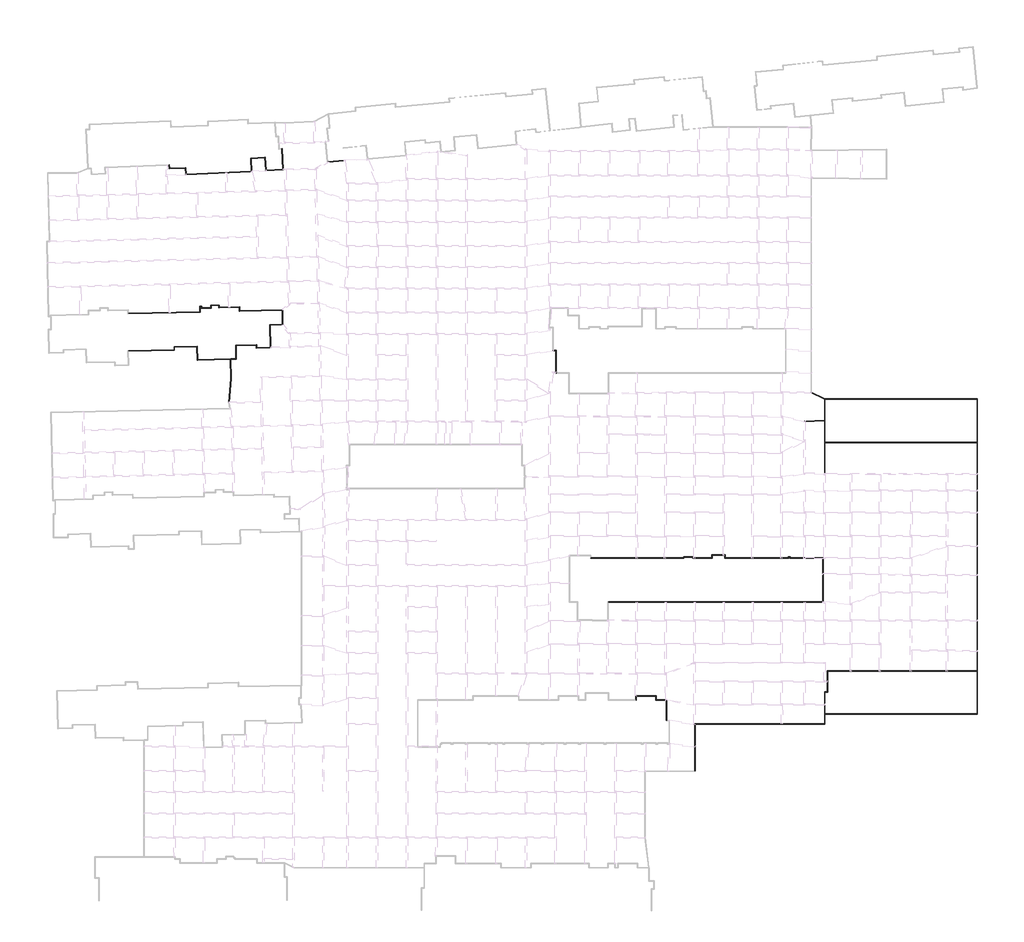
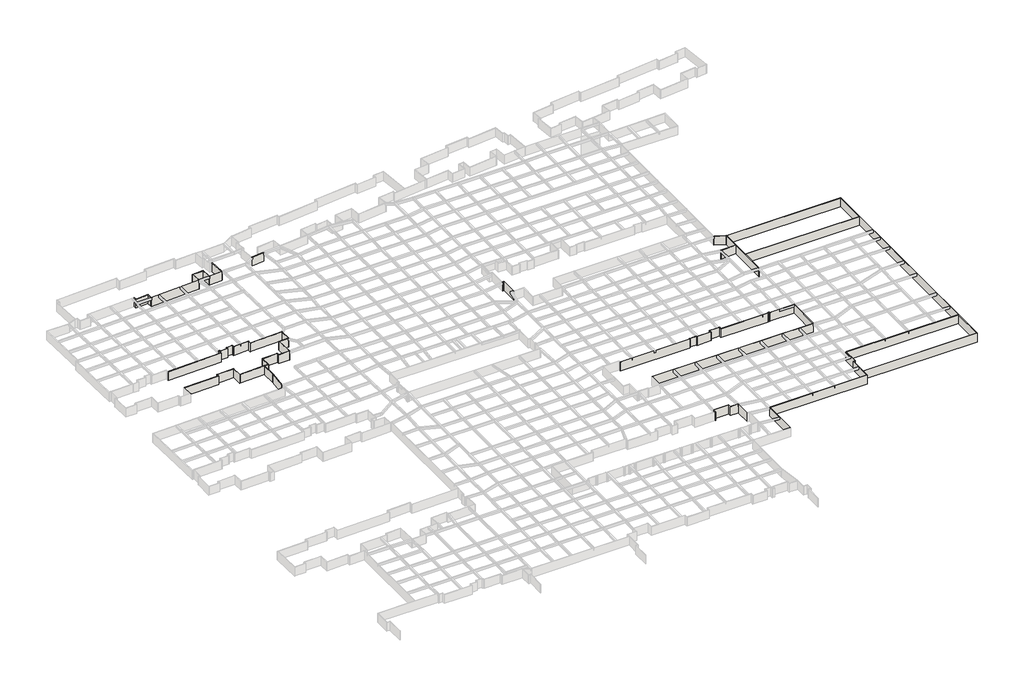
# One storey, part 5 of 20: 71 walls.
"""IFC4 building model written with IfcOpenShell, lengths in millimetres."""

from ifc_helpers import new_model, si_unit, origin, origin_with_axes, place, context, project, spatial, polyline, outline, extrude, faceted_brep, element, save

model = new_model("IFC4")

# Units and contexts
model_context = context("Model", 3, world=origin())
ifc_project = project(units=[si_unit("LENGTHUNIT", "METRE", prefix="MILLI")], contexts=[model_context])

# Site, building, storey
site = spatial("IfcSite", under=ifc_project)
building = spatial("IfcBuilding", under=site)
storey = spatial("IfcBuildingStorey", under=building, Name="户型图", Elevation=0.0)

# Walls
placement = place(None, origin())
element("IfcWall", 1, ObjectType="所有墙体", at=placement, inside=storey, context=model_context, shape_type="Brep", body=[
    faceted_brep([(-4228.4021072, 138757.8636225, 0.0), (8173.0072094, 139059.136348, 0.0), (8173.0072094, 139059.136348, 3300.0), (-4228.4021072, 138757.8636225, 3300.0), (-4231.3164585, 138877.8282279, 0.0), (-4231.3164585, 138877.8282279, 3300.0), (8053.0072094, 139176.2565418, 3300.0), (8173.0072094, 139179.171753, 3300.0), (8173.0072094, 139179.171753, 0.0), (8053.0072094, 139176.2565418, 0.0)], [[[0, 1, 2, 3]], [[4, 5, 6, 7, 8, 9]], [[1, 0, 4, 9, 8]], [[3, 2, 7, 6, 5]], [[0, 3, 5, 4]], [[2, 1, 8, 7]]]),
])
element("IfcWall", 2, ObjectType="所有墙体", at=placement, inside=storey, context=model_context, shape_type="Brep", body=[
    faceted_brep([(8173.0072094, 139179.171753, 0.0), (8173.0072094, 139859.136348, 0.0), (8173.0072094, 139979.171753, 0.0), (8173.0072094, 139979.171753, 3300.0), (8173.0072094, 139859.136348, 3300.0), (8173.0072094, 139179.171753, 3300.0), (8053.0072094, 139176.2565418, 0.0), (8053.0072094, 139176.2565418, 3300.0), (8053.0072094, 139976.2565418, 3300.0), (8053.0072094, 139976.2565418, 0.0)], [[[0, 1, 2, 3, 4, 5]], [[6, 7, 8, 9]], [[2, 1, 0, 6, 9]], [[5, 4, 3, 8, 7]], [[0, 5, 7, 6]], [[3, 2, 9, 8]]]),
])
element("IfcWall", 3, ObjectType="所有墙体", at=placement, inside=storey, context=model_context, shape_type="Brep", body=[
    faceted_brep([(8173.0072094, 139859.136348, 0.0), (14152.6828585, 140004.4031588, 0.0), (14272.6474639, 140007.3175101, 0.0), (14272.6474639, 140007.3175101, 3300.0), (14152.6828585, 140004.4031588, 3300.0), (8173.0072094, 139859.136348, 3300.0), (8173.0072094, 139979.171753, 0.0), (8173.0072094, 139979.171753, 3300.0), (14269.7331126, 140127.2821155, 3300.0), (14269.7331126, 140127.2821155, 0.0)], [[[0, 1, 2, 3, 4, 5]], [[6, 7, 8, 9]], [[2, 1, 0, 6, 9]], [[5, 4, 3, 8, 7]], [[0, 5, 7, 6]], [[3, 2, 9, 8]]]),
])
element("IfcWall", 4, ObjectType="所有墙体", at=placement, inside=storey, context=model_context, shape_type="Brep", body=[
    faceted_brep([(14152.6828585, 140004.4031588, 0.0), (14240.0810776, 136406.7954185, 0.0), (14240.0810776, 136406.7954185, 3300.0), (14152.6828585, 140004.4031588, 3300.0), (14272.6474639, 140007.3175101, 0.0), (14272.6474639, 140007.3175101, 3300.0), (14357.1313318, 136529.6743753, 3300.0), (14360.0456831, 136409.7097698, 3300.0), (14360.0456831, 136409.7097698, 0.0), (14357.1313318, 136529.6743753, 0.0)], [[[0, 1, 2, 3]], [[4, 5, 6, 7, 8, 9]], [[1, 0, 4, 9, 8]], [[3, 2, 7, 6, 5]], [[0, 3, 5, 4]], [[2, 1, 8, 7]]]),
])
element("IfcWall", 5, ObjectType="所有墙体", at=placement, inside=storey, context=model_context, shape_type="Brep", body=[
    faceted_brep([(14360.0456831, 136409.7097698, 0.0), (23216.491821, 136624.863193, 0.0), (23336.4564264, 136627.7775443, 0.0), (23336.4564264, 136627.7775443, 3300.0), (23216.491821, 136624.863193, 3300.0), (14360.0456831, 136409.7097698, 3300.0), (14357.1313318, 136529.6743753, 0.0), (14357.1313318, 136529.6743753, 3300.0), (23246.0635256, 136745.616996, 3300.0), (23333.5420751, 136747.7421497, 3300.0), (23333.5420751, 136747.7421497, 0.0), (23246.0635256, 136745.616996, 0.0), (23335.6240877, 136662.0394333, 0.0), (23335.6240877, 136662.0394333, 3300.0)], [[[0, 1, 2, 3, 4, 5]], [[6, 7, 8, 9, 10, 11]], [[2, 1, 0, 6, 11, 10, 12]], [[5, 4, 3, 13, 9, 8, 7]], [[0, 5, 7, 6]], [[3, 2, 12, 10, 9, 13]]]),
])
element("IfcWall", 6, ObjectType="所有墙体", at=placement, inside=storey, context=model_context, shape_type="SweptSolid", body=[
    extrude(outline(polyline([(23339.7846649, 131549.7107032), (23216.491821, 136624.863193), (23336.4564264, 136627.7775443), (23459.9119945, 131545.9267742), (23339.7846649, 131549.7107032)])), origin_with_axes(), (0.0, 0.0, 1.0), 3300.0),
])
element("IfcWall", 7, ObjectType="所有墙体", at=placement, inside=storey, context=model_context, shape_type="SweptSolid", body=[
    extrude(outline(polyline([(22764.2529371, 124971.3529529), (23339.7846649, 131549.7107032), (23459.9119945, 131545.9267742), (22884.987918, 124974.5145097), (22764.2529371, 124971.3529529)])), origin_with_axes(), (0.0, 0.0, 1.0), 3300.0),
])
element("IfcWall", 8, ObjectType="所有墙体", at=placement, inside=storey, context=model_context, shape_type="Brep", body=[
    faceted_brep([(148100.0, 25994.6126828, 0.0), (148100.0, 38580.0, 0.0), (148100.0, 38700.0, 0.0), (148100.0, 38700.0, 3300.0), (148100.0, 38580.0, 3300.0), (148100.0, 25994.6126828, 3300.0), (147980.0, 25994.6126828, 0.0), (147980.0, 25994.6126828, 3300.0), (147980.0, 38700.0, 3300.0), (147980.0, 38700.0, 0.0)], [[[0, 1, 2, 3, 4, 5]], [[6, 7, 8, 9]], [[2, 1, 0, 6, 9]], [[5, 4, 3, 8, 7]], [[0, 5, 7, 6]], [[3, 2, 9, 8]]]),
])
element("IfcWall", 9, ObjectType="所有墙体", at=placement, inside=storey, context=model_context, shape_type="Brep", body=[
    faceted_brep([(148100.0, 38580.0, 0.0), (182984.9999996, 38580.0, 0.0), (182984.9999996, 38580.0, 3300.0), (148100.0, 38580.0, 3300.0), (148100.0, 38700.0, 0.0), (148100.0, 38700.0, 3300.0), (182864.9999996, 38700.0, 3300.0), (182984.9999996, 38700.0, 3300.0), (182984.9999996, 38700.0, 0.0), (182864.9999996, 38700.0, 0.0)], [[[0, 1, 2, 3]], [[4, 5, 6, 7, 8, 9]], [[1, 0, 4, 9, 8]], [[3, 2, 7, 6, 5]], [[0, 3, 5, 4]], [[2, 1, 8, 7]]]),
])
element("IfcWall", 10, ObjectType="所有墙体", at=placement, inside=storey, context=model_context, shape_type="Brep", body=[
    faceted_brep([(182984.9999996, 38700.0, 0.0), (182984.9999996, 41206.0, 0.0), (182984.9999996, 41326.0, 0.0), (182984.9999996, 47205.0, 0.0), (182984.9999996, 47325.0, 0.0), (182984.9999996, 47325.0, 3300.0), (182984.9999996, 47205.0, 3300.0), (182984.9999996, 41326.0, 3300.0), (182984.9999996, 41206.0, 3300.0), (182984.9999996, 38700.0, 3300.0), (182864.9999996, 38700.0, 0.0), (182864.9999996, 38700.0, 3300.0), (182864.9999996, 47325.0, 3300.0), (182864.9999996, 47325.0, 0.0)], [[[0, 1, 2, 3, 4, 5, 6, 7, 8, 9]], [[10, 11, 12, 13]], [[4, 3, 2, 1, 0, 10, 13]], [[9, 8, 7, 6, 5, 12, 11]], [[0, 9, 11, 10]], [[5, 4, 13, 12]]]),
])
element("IfcWall", 11, ObjectType="所有墙体", at=placement, inside=storey, context=model_context, shape_type="Brep", body=[
    faceted_brep([(182984.9999996, 41206.0, 0.0), (223958.0, 41206.0, 0.0), (223958.0, 41206.0, 3300.0), (182984.9999996, 41206.0, 3300.0), (182984.9999996, 41326.0, 0.0), (182984.9999996, 41326.0, 3300.0), (223838.0, 41326.0, 3300.0), (223958.0, 41326.0, 3300.0), (223958.0, 41326.0, 0.0), (223838.0, 41326.0, 0.0)], [[[0, 1, 2, 3]], [[4, 5, 6, 7, 8, 9]], [[1, 0, 4, 9, 8]], [[3, 2, 7, 6, 5]], [[0, 3, 5, 4]], [[2, 1, 8, 7]]]),
])
element("IfcWall", 12, ObjectType="所有墙体", at=placement, inside=storey, context=model_context, shape_type="Brep", body=[
    faceted_brep([(223958.0, 41326.0, 0.0), (223958.0, 126084.0, 0.0), (223958.0, 126084.0, 3300.0), (223958.0, 41326.0, 3300.0), (223838.0, 41326.0, 0.0), (223838.0, 41326.0, 3300.0), (223838.0, 52805.0, 3300.0), (223838.0, 52925.0, 3300.0), (223838.0, 114264.0, 3300.0), (223838.0, 114384.0, 3300.0), (223838.0, 125964.0, 3300.0), (223838.0, 126084.0, 3300.0), (223838.0, 126084.0, 0.0), (223838.0, 125964.0, 0.0), (223838.0, 114384.0, 0.0), (223838.0, 114264.0, 0.0), (223838.0, 52925.0, 0.0), (223838.0, 52805.0, 0.0)], [[[0, 1, 2, 3]], [[4, 5, 6, 7, 8, 9, 10, 11, 12, 13, 14, 15, 16, 17]], [[1, 0, 4, 17, 16, 15, 14, 13, 12]], [[3, 2, 11, 10, 9, 8, 7, 6, 5]], [[0, 3, 5, 4]], [[2, 1, 12, 11]]]),
])
element("IfcWall", 13, ObjectType="所有墙体", at=placement, inside=storey, context=model_context, shape_type="Brep", body=[
    faceted_brep([(223838.0, 126084.0, 0.0), (182938.3016794, 126084.0, 0.0), (182654.3574894, 126084.0, 0.0), (182654.3574894, 126084.0, 3300.0), (182938.3016794, 126084.0, 3300.0), (223838.0, 126084.0, 3300.0), (223838.0, 125964.0, 0.0), (223838.0, 125964.0, 3300.0), (182984.9999996, 125964.0, 3300.0), (182911.6983199, 125964.0, 3300.0), (182911.6983199, 125964.0, 0.0), (182984.9999996, 125964.0, 0.0), (182864.9999996, 125985.7757844, 0.0), (182864.9999996, 125985.7757844, 3300.0)], [[[0, 1, 2, 3, 4, 5]], [[6, 7, 8, 9, 10, 11]], [[2, 1, 0, 6, 11, 10, 12]], [[5, 4, 3, 13, 9, 8, 7]], [[0, 5, 7, 6]], [[3, 2, 12, 10, 9, 13]]]),
])
element("IfcWall", 14, ObjectType="所有墙体", at=placement, inside=storey, context=model_context, shape_type="Brep", body=[
    faceted_brep([(182938.3016794, 126084.0, 0.0), (179359.7688515, 127752.6972626, 0.0), (179239.7688515, 127808.6541816, 0.0), (179239.7688515, 127808.6541816, 3300.0), (179359.7688515, 127752.6972626, 3300.0), (182938.3016794, 126084.0, 3300.0), (182654.3574894, 126084.0, 0.0), (182654.3574894, 126084.0, 3300.0), (179239.7688515, 127676.2488313, 3300.0), (179239.7688515, 127676.2488313, 0.0)], [[[0, 1, 2, 3, 4, 5]], [[6, 7, 8, 9]], [[2, 1, 0, 6, 9]], [[5, 4, 3, 8, 7]], [[0, 5, 7, 6]], [[3, 2, 9, 8]]]),
])
element("IfcWall", 15, ObjectType="所有墙体", at=placement, inside=storey, context=model_context, shape_type="SweptSolid", body=[
    extrude(outline(polyline([(53846.8616542, 190018.1389708), (49331.2355692, 189543.5275444), (49319.6896824, 189662.9750163), (53834.3182386, 190137.4815982), (53846.8616542, 190018.1389708)])), origin_with_axes(), (0.0, 0.0, 1.0), 3300.0),
])
element("IfcWall", 16, ObjectType="所有墙体", at=placement, inside=storey, context=model_context, shape_type="Brep", body=[
    faceted_brep([(37019.504808, 193167.4722862, 0.0), (37309.4460056, 187635.0646637, 0.0), (37315.7263203, 187515.2291195, 0.0), (37315.7263203, 187515.2291195, 3300.0), (37309.4460056, 187635.0646637, 3300.0), (37019.504808, 193167.4722862, 3300.0), (37139.3403522, 193173.752601, 0.0), (37139.3403522, 193173.752601, 3300.0), (37435.5618645, 187521.5094342, 3300.0), (37435.5618645, 187521.5094342, 0.0)], [[[0, 1, 2, 3, 4, 5]], [[6, 7, 8, 9]], [[2, 1, 0, 6, 9]], [[5, 4, 3, 8, 7]], [[0, 5, 7, 6]], [[3, 2, 9, 8]]]),
])
element("IfcWall", 17, ObjectType="所有墙体", at=placement, inside=storey, context=model_context, shape_type="Brep", body=[
    faceted_brep([(37309.4460056, 187635.0646637, 0.0), (32786.9007673, 187398.048111, 0.0), (32667.0652231, 187391.7677963, 0.0), (32667.0652231, 187391.7677963, 3300.0), (32786.9007673, 187398.048111, 3300.0), (37309.4460056, 187635.0646637, 3300.0), (37315.7263203, 187515.2291195, 0.0), (37315.7263203, 187515.2291195, 3300.0), (32793.1810821, 187278.2125669, 3300.0), (32673.3455379, 187271.9322521, 3300.0), (32673.3455379, 187271.9322521, 2500.0), (32673.3455379, 187271.9322521, 0.0)], [[[0, 1, 2, 3, 4, 5]], [[6, 7, 8, 9, 10, 11]], [[2, 1, 0, 6, 11]], [[5, 4, 3, 9, 8, 7]], [[0, 5, 7, 6]], [[3, 2, 11, 10, 9]]]),
])
element("IfcWall", 18, ObjectType="所有墙体", at=placement, inside=storey, context=model_context, shape_type="Brep", body=[
    faceted_brep([(32786.9007673, 187398.048111, 0.0), (32602.4342162, 190917.8795872, 0.0), (32602.4342162, 190917.8795872, 3300.0), (32786.9007673, 187398.048111, 3300.0), (32667.0652231, 187391.7677963, 0.0), (32667.0652231, 187391.7677963, 3300.0), (32488.8789868, 190791.7637283, 3300.0), (32482.598672, 190911.5992725, 3300.0), (32482.598672, 190911.5992725, 0.0), (32488.8789868, 190791.7637283, 0.0)], [[[0, 1, 2, 3]], [[4, 5, 6, 7, 8, 9]], [[1, 0, 4, 9, 8]], [[3, 2, 7, 6, 5]], [[0, 3, 5, 4]], [[2, 1, 8, 7]]]),
])
element("IfcWall", 19, ObjectType="所有墙体", at=placement, inside=storey, context=model_context, shape_type="Brep", body=[
    faceted_brep([(32482.598672, 190911.5992725, 0.0), (28607.9160772, 190708.5357622, 0.0), (28607.9160772, 190708.5357622, 3300.0), (32482.598672, 190911.5992725, 3300.0), (32488.8789868, 190791.7637283, 0.0), (32488.8789868, 190791.7637283, 3300.0), (28734.0319361, 190594.9805328, 3300.0), (28614.1963919, 190588.7002181, 3300.0), (28614.1963919, 190588.7002181, 0.0), (28734.0319361, 190594.9805328, 0.0)], [[[0, 1, 2, 3]], [[4, 5, 6, 7, 8, 9]], [[1, 0, 4, 9, 8]], [[3, 2, 7, 6, 5]], [[0, 3, 5, 4]], [[2, 1, 8, 7]]]),
])
element("IfcWall", 20, ObjectType="所有墙体", at=placement, inside=storey, context=model_context, shape_type="Brep", body=[
    faceted_brep([(28614.1963919, 190588.7002181, 0.0), (28794.7279523, 187143.9528373, 0.0), (28801.0084588, 187024.1136344, 0.0), (28801.0084588, 187024.1136344, 3300.0), (28794.7279523, 187143.9528373, 3300.0), (28614.1963919, 190588.7002181, 3300.0), (28734.0319361, 190594.9805328, 0.0), (28734.0319361, 190594.9805328, 3300.0), (28920.893079, 187029.4575233, 3300.0), (28920.893079, 187029.4575233, 0.0)], [[[0, 1, 2, 3, 4, 5]], [[6, 7, 8, 9]], [[2, 1, 0, 6, 9]], [[5, 4, 3, 8, 7]], [[0, 5, 7, 6]], [[3, 2, 9, 8]]]),
])
element("IfcWall", 21, ObjectType="所有墙体", at=placement, inside=storey, context=model_context, shape_type="Brep", body=[
    faceted_brep([(28794.7279523, 187143.9528373, 0.0), (11317.4343518, 186364.8978146, 0.0), (11197.5533917, 186359.5540888, 0.0), (11197.5533917, 186359.5540888, 3300.0), (11317.4343518, 186364.8978146, 3300.0), (28794.7279523, 187143.9528373, 3300.0), (28801.0084588, 187024.1136344, 0.0), (28801.0084588, 187024.1136344, 3300.0), (11322.7780776, 186245.0168545, 3300.0), (11202.8971175, 186239.6731287, 3300.0), (11202.8971175, 186239.6731287, 2500.0), (11202.8971175, 186239.6731287, 0.0)], [[[0, 1, 2, 3, 4, 5]], [[6, 7, 8, 9, 10, 11]], [[2, 1, 0, 6, 11]], [[5, 4, 3, 9, 8, 7]], [[0, 5, 7, 6]], [[3, 2, 11, 10, 9]]]),
])
element("IfcWall", 22, ObjectType="所有墙体", at=placement, inside=storey, context=model_context, shape_type="Brep", body=[
    faceted_brep([(11317.4343518, 186364.8978146, 0.0), (11237.3451707, 188161.6157523, 0.0), (11237.3451707, 188161.6157523, 3300.0), (11317.4343518, 186364.8978146, 3300.0), (11197.5533917, 186359.5540888, 0.0), (11197.5533917, 186359.5540888, 3300.0), (11122.8079363, 188036.3910664, 3300.0), (11117.4642106, 188156.2720265, 3300.0), (11117.4642106, 188156.2720265, 0.0), (11122.8079363, 188036.3910664, 0.0)], [[[0, 1, 2, 3]], [[4, 5, 6, 7, 8, 9]], [[1, 0, 4, 9, 8]], [[3, 2, 7, 6, 5]], [[0, 3, 5, 4]], [[2, 1, 8, 7]]]),
])
element("IfcWall", 23, ObjectType="所有墙体", at=placement, inside=storey, context=model_context, shape_type="Brep", body=[
    faceted_brep([(11117.4642106, 188156.2720265, 0.0), (6836.276518, 187965.4369435, 0.0), (6716.3955579, 187960.0932177, 0.0), (6716.3955579, 187960.0932177, 3300.0), (6836.276518, 187965.4369435, 3300.0), (11117.4642106, 188156.2720265, 3300.0), (11122.8079363, 188036.3910664, 0.0), (11122.8079363, 188036.3910664, 3300.0), (6721.7392837, 187840.2122576, 3300.0), (6721.7392837, 187840.2122576, 0.0)], [[[0, 1, 2, 3, 4, 5]], [[6, 7, 8, 9]], [[2, 1, 0, 6, 9]], [[5, 4, 3, 8, 7]], [[0, 5, 7, 6]], [[3, 2, 9, 8]]]),
])
element("IfcWall", 24, ObjectType="所有墙体", at=placement, inside=storey, context=model_context, shape_type="Brep", body=[
    faceted_brep([(6836.276518, 187965.4369435, 0.0), (6791.7370894, 188964.6329557, 0.0), (6791.7370894, 188964.6329557, 3300.0), (6836.276518, 187965.4369435, 3300.0), (6716.3955579, 187960.0932177, 0.0), (6716.3955579, 187960.0932177, 3300.0), (6677.199855, 188839.4082698, 3300.0), (6671.8561293, 188959.2892299, 3300.0), (6671.8561293, 188959.2892299, 0.0), (6677.199855, 188839.4082698, 0.0)], [[[0, 1, 2, 3]], [[4, 5, 6, 7, 8, 9]], [[1, 0, 4, 9, 8]], [[3, 2, 7, 6, 5]], [[0, 3, 5, 4]], [[2, 1, 8, 7]]]),
])
element("IfcWall", 25, ObjectType="所有墙体", at=placement, inside=storey, context=model_context, shape_type="Brep", body=[
    faceted_brep([(109995.8712071, 138929.7156576, 0.0), (110579.0, 138929.7156576, 0.0), (110699.0, 138929.7156576, 0.0), (110699.0, 138929.7156576, 3300.0), (110579.0, 138929.7156576, 3300.0), (109995.8712071, 138929.7156576, 3300.0), (109995.8712071, 139049.7156576, 0.0), (109995.8712071, 139049.7156576, 3300.0), (110699.0, 139049.7156576, 3300.0), (110699.0, 139049.7156576, 0.0)], [[[0, 1, 2, 3, 4, 5]], [[6, 7, 8, 9]], [[2, 1, 0, 6, 9]], [[5, 4, 3, 8, 7]], [[0, 5, 7, 6]], [[3, 2, 9, 8]]]),
])
element("IfcWall", 26, ObjectType="所有墙体", at=placement, inside=storey, context=model_context, shape_type="Brep", body=[
    faceted_brep([(110579.0, 138929.7156576, 0.0), (110579.0, 132933.0, 0.0), (110579.0, 132933.0, 3300.0), (110579.0, 138929.7156576, 3300.0), (110699.0, 138929.7156576, 0.0), (110699.0, 138929.7156576, 3300.0), (110699.0, 133053.0, 3300.0), (110699.0, 132933.0, 3300.0), (110699.0, 132933.0, 0.0), (110699.0, 133053.0, 0.0)], [[[0, 1, 2, 3]], [[4, 5, 6, 7, 8, 9]], [[1, 0, 4, 9, 8]], [[3, 2, 7, 6, 5]], [[0, 3, 5, 4]], [[2, 1, 8, 7]]]),
])
element("IfcWall", 27, ObjectType="所有墙体", at=placement, inside=storey, context=model_context, shape_type="Brep", body=[
    faceted_brep([(182864.9999996, 125985.7757844, 0.0), (182864.9999996, 120234.5396241, 0.0), (182864.9999996, 120114.471487, 0.0), (182864.9999996, 105802.5076858, 0.0), (182864.9999996, 105802.5076858, 3300.0), (182864.9999996, 120114.471487, 3300.0), (182864.9999996, 120234.5396241, 3300.0), (182864.9999996, 125985.7757844, 3300.0), (182984.9999996, 125964.0, 0.0), (182984.9999996, 125964.0, 3300.0), (182984.9999996, 114384.0, 3300.0), (182984.9999996, 114264.0, 3300.0), (182984.9999996, 105802.5076858, 3300.0), (182984.9999996, 105802.5076858, 0.0), (182984.9999996, 114264.0, 0.0), (182984.9999996, 114384.0, 0.0), (182911.6983199, 125964.0, 0.0), (182911.6983199, 125964.0, 3300.0)], [[[0, 1, 2, 3, 4, 5, 6, 7]], [[8, 9, 10, 11, 12, 13, 14, 15]], [[3, 2, 1, 0, 16, 8, 15, 14, 13]], [[4, 3, 13, 12]], [[7, 6, 5, 4, 12, 11, 10, 9, 17]], [[0, 7, 17, 16]], [[17, 9, 8, 16]]]),
])
element("IfcWall", 28, ObjectType="所有墙体", at=placement, inside=storey, context=model_context, shape_type="SweptSolid", body=[
    extrude(outline(polyline([(223838.0, 114264.0), (182984.9999996, 114264.0), (182984.9999996, 114384.0), (223838.0, 114384.0), (223838.0, 114264.0)])), origin_with_axes(), (0.0, 0.0, 1.0), 3300.0),
])
element("IfcWall", 29, ObjectType="所有墙体", at=placement, inside=storey, context=model_context, shape_type="SweptSolid", body=[
    extrude(outline(polyline([(182864.9999996, 120114.471487), (177452.0210746, 119932.0340492), (177447.9789254, 120051.9659508), (182864.9999996, 120234.5396241), (182864.9999996, 120114.471487)])), origin_with_axes(), (0.0, 0.0, 1.0), 3300.0),
])
element("IfcWall", 30, ObjectType="所有墙体", at=placement, inside=storey, context=model_context, shape_type="Brep", body=[
    faceted_brep([(124710.0, 71310.0, 0.0), (182496.0, 71310.0, 0.0), (182496.0, 71310.0, 3300.0), (124710.0, 71310.0, 3300.0), (124710.0, 71430.0, 0.0), (124710.0, 71430.0, 3300.0), (182376.0, 71430.0, 3300.0), (182496.0, 71430.0, 3300.0), (182496.0, 71430.0, 0.0), (182376.0, 71430.0, 0.0)], [[[0, 1, 2, 3]], [[4, 5, 6, 7, 8, 9]], [[1, 0, 4, 9, 8]], [[3, 2, 7, 6, 5]], [[0, 3, 5, 4]], [[2, 1, 8, 7]]]),
])
element("IfcWall", 31, ObjectType="所有墙体", at=placement, inside=storey, context=model_context, shape_type="Brep", body=[
    faceted_brep([(182496.0, 71430.0, 0.0), (182496.0, 83280.0, 0.0), (182496.0, 83280.0, 3300.0), (182496.0, 71430.0, 3300.0), (182376.0, 71430.0, 0.0), (182376.0, 71430.0, 3300.0), (182376.0, 83160.0, 3300.0), (182376.0, 83280.0, 3300.0), (182376.0, 83280.0, 0.0), (182376.0, 83160.0, 0.0)], [[[0, 1, 2, 3]], [[4, 5, 6, 7, 8, 9]], [[1, 0, 4, 9, 8]], [[3, 2, 7, 6, 5]], [[0, 3, 5, 4]], [[2, 1, 8, 7]]]),
])
element("IfcWall", 32, ObjectType="所有墙体", at=placement, inside=storey, context=model_context, shape_type="SweptSolid", body=[
    extrude(outline(polyline([(173697.0, 83280.0), (182376.0, 83280.0), (182376.0, 83160.0), (173697.0, 83160.0), (173697.0, 83280.0)])), origin_with_axes(), (0.0, 0.0, 1.0), 3300.0),
])
element("IfcWall", 33, ObjectType="所有墙体", at=placement, inside=storey, context=model_context, shape_type="Brep", body=[
    faceted_brep([(173697.0, 83160.0, 0.0), (173697.0, 83280.0, 0.0), (173697.0, 83530.0, 0.0), (173697.0, 83530.0, 3300.0), (173697.0, 83280.0, 3300.0), (173697.0, 83160.0, 3300.0), (173577.0, 83160.0, 0.0), (173577.0, 83160.0, 3300.0), (173577.0, 83410.0, 3300.0), (173577.0, 83530.0, 3300.0), (173577.0, 83530.0, 0.0), (173577.0, 83410.0, 0.0)], [[[0, 1, 2, 3, 4, 5]], [[6, 7, 8, 9, 10, 11]], [[2, 1, 0, 6, 11, 10]], [[5, 4, 3, 9, 8, 7]], [[0, 5, 7, 6]], [[3, 2, 10, 9]]]),
])
element("IfcWall", 34, ObjectType="所有墙体", at=placement, inside=storey, context=model_context, shape_type="SweptSolid", body=[
    extrude(outline(polyline([(173197.0, 83530.0), (173577.0, 83530.0), (173577.0, 83410.0), (173197.0, 83410.0), (173197.0, 83530.0)])), origin_with_axes(), (0.0, 0.0, 1.0), 3300.0),
])
element("IfcWall", 35, ObjectType="所有墙体", at=placement, inside=storey, context=model_context, shape_type="Brep", body=[
    faceted_brep([(173077.0, 83530.0, 0.0), (173077.0, 83280.0, 0.0), (173077.0, 83160.0, 0.0), (173077.0, 83160.0, 3300.0), (173077.0, 83280.0, 3300.0), (173077.0, 83530.0, 3300.0), (173197.0, 83530.0, 0.0), (173197.0, 83530.0, 3300.0), (173197.0, 83410.0, 3300.0), (173197.0, 83160.0, 3300.0), (173197.0, 83160.0, 0.0), (173197.0, 83410.0, 0.0)], [[[0, 1, 2, 3, 4, 5]], [[6, 7, 8, 9, 10, 11]], [[2, 1, 0, 6, 11, 10]], [[5, 4, 3, 9, 8, 7]], [[0, 5, 7, 6]], [[3, 2, 10, 9]]]),
])
element("IfcWall", 36, ObjectType="所有墙体", at=placement, inside=storey, context=model_context, shape_type="Brep", body=[
    faceted_brep([(173077.0, 83280.0, 0.0), (156196.0, 83280.0, 0.0), (156076.0, 83280.0, 0.0), (156076.0, 83280.0, 3300.0), (156196.0, 83280.0, 3300.0), (173077.0, 83280.0, 3300.0), (173077.0, 83160.0, 0.0), (173077.0, 83160.0, 3300.0), (156076.0, 83160.0, 3300.0), (156076.0, 83160.0, 0.0)], [[[0, 1, 2, 3, 4, 5]], [[6, 7, 8, 9]], [[2, 1, 0, 6, 9]], [[5, 4, 3, 8, 7]], [[0, 5, 7, 6]], [[3, 2, 9, 8]]]),
])
element("IfcWall", 37, ObjectType="所有墙体", at=placement, inside=storey, context=model_context, shape_type="Brep", body=[
    faceted_brep([(156196.0, 83280.0, 0.0), (156196.0, 84080.0, 0.0), (156196.0, 84080.0, 3300.0), (156196.0, 83280.0, 3300.0), (156076.0, 83280.0, 0.0), (156076.0, 83280.0, 3300.0), (156076.0, 83960.0, 3300.0), (156076.0, 84080.0, 3300.0), (156076.0, 84080.0, 0.0), (156076.0, 83960.0, 0.0)], [[[0, 1, 2, 3]], [[4, 5, 6, 7, 8, 9]], [[1, 0, 4, 9, 8]], [[3, 2, 7, 6, 5]], [[0, 3, 5, 4]], [[2, 1, 8, 7]]]),
])
element("IfcWall", 38, ObjectType="所有墙体", at=placement, inside=storey, context=model_context, shape_type="Brep", body=[
    faceted_brep([(156076.0, 84080.0, 0.0), (152569.0, 84080.0, 0.0), (152569.0, 84080.0, 3300.0), (156076.0, 84080.0, 3300.0), (156076.0, 83960.0, 0.0), (156076.0, 83960.0, 3300.0), (152689.0, 83960.0, 3300.0), (152569.0, 83960.0, 3300.0), (152569.0, 83960.0, 0.0), (152689.0, 83960.0, 0.0)], [[[0, 1, 2, 3]], [[4, 5, 6, 7, 8, 9]], [[1, 0, 4, 9, 8]], [[3, 2, 7, 6, 5]], [[0, 3, 5, 4]], [[2, 1, 8, 7]]]),
])
element("IfcWall", 39, ObjectType="所有墙体", at=placement, inside=storey, context=model_context, shape_type="Brep", body=[
    faceted_brep([(152569.0, 83960.0, 0.0), (152569.0, 83280.0, 0.0), (152569.0, 83160.0, 0.0), (152569.0, 83160.0, 3300.0), (152569.0, 83280.0, 3300.0), (152569.0, 83960.0, 3300.0), (152689.0, 83960.0, 0.0), (152689.0, 83960.0, 3300.0), (152689.0, 83160.0, 3300.0), (152689.0, 83160.0, 0.0)], [[[0, 1, 2, 3, 4, 5]], [[6, 7, 8, 9]], [[2, 1, 0, 6, 9]], [[5, 4, 3, 8, 7]], [[0, 5, 7, 6]], [[3, 2, 9, 8]]]),
])
element("IfcWall", 40, ObjectType="所有墙体", at=placement, inside=storey, context=model_context, shape_type="SweptSolid", body=[
    extrude(outline(polyline([(147597.0, 83280.0), (152569.0, 83280.0), (152569.0, 83160.0), (147597.0, 83160.0), (147597.0, 83280.0)])), origin_with_axes(), (0.0, 0.0, 1.0), 3300.0),
])
element("IfcWall", 41, ObjectType="所有墙体", at=placement, inside=storey, context=model_context, shape_type="Brep", body=[
    faceted_brep([(147597.0, 83160.0, 0.0), (147597.0, 83280.0, 0.0), (147597.0, 83530.0, 0.0), (147597.0, 83530.0, 3300.0), (147597.0, 83280.0, 3300.0), (147597.0, 83160.0, 3300.0), (147477.0, 83160.0, 0.0), (147477.0, 83160.0, 3300.0), (147477.0, 83410.0, 3300.0), (147477.0, 83530.0, 3300.0), (147477.0, 83530.0, 0.0), (147477.0, 83410.0, 0.0)], [[[0, 1, 2, 3, 4, 5]], [[6, 7, 8, 9, 10, 11]], [[2, 1, 0, 6, 11, 10]], [[5, 4, 3, 9, 8, 7]], [[0, 5, 7, 6]], [[3, 2, 10, 9]]]),
])
element("IfcWall", 42, ObjectType="所有墙体", at=placement, inside=storey, context=model_context, shape_type="SweptSolid", body=[
    extrude(outline(polyline([(145095.0, 83530.0), (147477.0, 83530.0), (147477.0, 83410.0), (145095.0, 83410.0), (145095.0, 83530.0)])), origin_with_axes(), (0.0, 0.0, 1.0), 3300.0),
])
element("IfcWall", 43, ObjectType="所有墙体", at=placement, inside=storey, context=model_context, shape_type="Brep", body=[
    faceted_brep([(144975.0, 83530.0, 0.0), (144975.0, 83280.0, 0.0), (144975.0, 83160.0, 0.0), (144975.0, 83160.0, 3300.0), (144975.0, 83280.0, 3300.0), (144975.0, 83530.0, 3300.0), (145095.0, 83530.0, 0.0), (145095.0, 83530.0, 3300.0), (145095.0, 83410.0, 3300.0), (145095.0, 83160.0, 3300.0), (145095.0, 83160.0, 0.0), (145095.0, 83410.0, 0.0)], [[[0, 1, 2, 3, 4, 5]], [[6, 7, 8, 9, 10, 11]], [[2, 1, 0, 6, 11, 10]], [[5, 4, 3, 9, 8, 7]], [[0, 5, 7, 6]], [[3, 2, 10, 9]]]),
])
element("IfcWall", 44, ObjectType="所有墙体", at=placement, inside=storey, context=model_context, shape_type="Brep", body=[
    faceted_brep([(144975.0, 83280.0, 0.0), (120097.0, 83280.0, 0.0), (119977.0, 83280.0, 0.0), (119977.0, 83280.0, 3300.0), (120097.0, 83280.0, 3300.0), (144975.0, 83280.0, 3300.0), (144975.0, 83160.0, 0.0), (144975.0, 83160.0, 3300.0), (119977.0, 83160.0, 3300.0), (119977.0, 83160.0, 0.0)], [[[0, 1, 2, 3, 4, 5]], [[6, 7, 8, 9]], [[2, 1, 0, 6, 9]], [[5, 4, 3, 8, 7]], [[0, 5, 7, 6]], [[3, 2, 9, 8]]]),
])
element("IfcWall", 45, ObjectType="所有墙体", at=placement, inside=storey, context=model_context, shape_type="Brep", body=[
    faceted_brep([(140504.0, 39568.0, 0.0), (140504.0, 45158.2500378, 0.0), (140504.0, 45158.2500378, 3300.0), (140504.0, 39568.0, 3300.0), (140384.0, 39568.0, 0.0), (140384.0, 39568.0, 3300.0), (140384.0, 45038.2500378, 3300.0), (140384.0, 45158.2500378, 3300.0), (140384.0, 45158.2500378, 0.0), (140384.0, 45038.2500378, 0.0)], [[[0, 1, 2, 3]], [[4, 5, 6, 7, 8, 9]], [[1, 0, 4, 9, 8]], [[3, 2, 7, 6, 5]], [[0, 3, 5, 4]], [[2, 1, 8, 7]]]),
])
element("IfcWall", 46, ObjectType="所有墙体", at=placement, inside=storey, context=model_context, shape_type="Brep", body=[
    faceted_brep([(140384.0, 45158.2500378, 0.0), (137604.0, 45158.2500378, 0.0), (137484.0, 45158.2500378, 0.0), (137484.0, 45158.2500378, 3300.0), (137604.0, 45158.2500378, 3300.0), (140384.0, 45158.2500378, 3300.0), (140384.0, 45038.2500378, 0.0), (140384.0, 45038.2500378, 3300.0), (137484.0, 45038.2500378, 3300.0), (137484.0, 45038.2500378, 0.0)], [[[0, 1, 2, 3, 4, 5]], [[6, 7, 8, 9]], [[2, 1, 0, 6, 9]], [[5, 4, 3, 8, 7]], [[0, 5, 7, 6]], [[3, 2, 9, 8]]]),
])
element("IfcWall", 47, ObjectType="所有墙体", at=placement, inside=storey, context=model_context, shape_type="Brep", body=[
    faceted_brep([(137604.0, 45158.2500378, 0.0), (137604.0, 46218.0, 0.0), (137604.0, 46218.0, 3300.0), (137604.0, 45158.2500378, 3300.0), (137484.0, 45158.2500378, 0.0), (137484.0, 45158.2500378, 3300.0), (137484.0, 46098.0, 3300.0), (137484.0, 46218.0, 3300.0), (137484.0, 46218.0, 0.0), (137484.0, 46098.0, 0.0)], [[[0, 1, 2, 3]], [[4, 5, 6, 7, 8, 9]], [[1, 0, 4, 9, 8]], [[3, 2, 7, 6, 5]], [[0, 3, 5, 4]], [[2, 1, 8, 7]]]),
])
element("IfcWall", 48, ObjectType="所有墙体", at=placement, inside=storey, context=model_context, shape_type="Brep", body=[
    faceted_brep([(137484.0, 46218.0, 0.0), (132088.0, 46218.0, 0.0), (132088.0, 46218.0, 3300.0), (137484.0, 46218.0, 3300.0), (137484.0, 46098.0, 0.0), (137484.0, 46098.0, 3300.0), (132208.0, 46098.0, 3300.0), (132088.0, 46098.0, 3300.0), (132088.0, 46098.0, 0.0), (132208.0, 46098.0, 0.0)], [[[0, 1, 2, 3]], [[4, 5, 6, 7, 8, 9]], [[1, 0, 4, 9, 8]], [[3, 2, 7, 6, 5]], [[0, 3, 5, 4]], [[2, 1, 8, 7]]]),
])
element("IfcWall", 49, ObjectType="所有墙体", at=placement, inside=storey, context=model_context, shape_type="Brep", body=[
    faceted_brep([(132088.0, 46098.0, 0.0), (132088.0, 45158.2500378, 0.0), (132088.0, 45038.2500378, 0.0), (132088.0, 45038.2500378, 3300.0), (132088.0, 45158.2500378, 3300.0), (132088.0, 46098.0, 3300.0), (132208.0, 46098.0, 0.0), (132208.0, 46098.0, 3300.0), (132208.0, 45038.2500378, 3300.0), (132208.0, 45038.2500378, 0.0)], [[[0, 1, 2, 3, 4, 5]], [[6, 7, 8, 9]], [[2, 1, 0, 6, 9]], [[5, 4, 3, 8, 7]], [[0, 5, 7, 6]], [[3, 2, 9, 8]]]),
])
element("IfcWall", 50, ObjectType="所有墙体", at=placement, inside=storey, context=model_context, shape_type="Brep", body=[
    faceted_brep([(-4259.3406744, 148854.8639982, 0.0), (15034.9666992, 149323.588836, 0.0), (15034.9666992, 149323.588836, 3300.0), (-4259.3406744, 148854.8639982, 3300.0), (-4259.3406744, 148974.8994033, 0.0), (-4259.3406744, 148974.8994033, 3300.0), (14914.9666992, 149440.7090298, 3300.0), (15034.9666992, 149443.624241, 3300.0), (15034.9666992, 149443.624241, 0.0), (14914.9666992, 149440.7090298, 0.0)], [[[0, 1, 2, 3]], [[4, 5, 6, 7, 8, 9]], [[1, 0, 4, 9, 8]], [[3, 2, 7, 6, 5]], [[0, 3, 5, 4]], [[2, 1, 8, 7]]]),
])
element("IfcWall", 51, ObjectType="所有墙体", at=placement, inside=storey, context=model_context, shape_type="Brep", body=[
    faceted_brep([(15034.9666992, 149443.624241, 0.0), (15034.9666992, 150722.1489329, 0.0), (15034.9666992, 150842.1489329, 0.0), (15034.9666992, 150842.1489329, 3300.0), (15034.9666992, 150722.1489329, 3300.0), (15034.9666992, 149443.624241, 3300.0), (14914.9666992, 149440.7090298, 0.0), (14914.9666992, 149440.7090298, 3300.0), (14914.9666992, 150842.1489329, 3300.0), (14914.9666992, 150842.1489329, 0.0)], [[[0, 1, 2, 3, 4, 5]], [[6, 7, 8, 9]], [[2, 1, 0, 6, 9]], [[5, 4, 3, 8, 7]], [[0, 5, 7, 6]], [[3, 2, 9, 8]]]),
])
element("IfcWall", 52, ObjectType="所有墙体", at=placement, inside=storey, context=model_context, shape_type="Brep", body=[
    faceted_brep([(15034.9666992, 150722.1489329, 0.0), (15322.0044256, 150722.1489329, 0.0), (15442.0044256, 150722.1489329, 0.0), (15442.0044256, 150722.1489329, 3300.0), (15322.0044256, 150722.1489329, 3300.0), (15034.9666992, 150722.1489329, 3300.0), (15034.9666992, 150842.1489329, 0.0), (15034.9666992, 150842.1489329, 3300.0), (15442.0044256, 150842.1489329, 3300.0), (15442.0044256, 150842.1489329, 0.0)], [[[0, 1, 2, 3, 4, 5]], [[6, 7, 8, 9]], [[2, 1, 0, 6, 9]], [[5, 4, 3, 8, 7]], [[0, 5, 7, 6]], [[3, 2, 9, 8]]]),
])
element("IfcWall", 53, ObjectType="所有墙体", at=placement, inside=storey, context=model_context, shape_type="SweptSolid", body=[
    extrude(outline(polyline([(15322.0044256, 150518.560744), (15322.0044256, 150722.1489329), (15442.0044256, 150722.1489329), (15442.0044256, 150518.560744), (15322.0044256, 150518.560744)])), origin_with_axes(), (0.0, 0.0, 1.0), 3300.0),
])
element("IfcWall", 54, ObjectType="所有墙体", at=placement, inside=storey, context=model_context, shape_type="Brep", body=[
    faceted_brep([(15322.0044256, 150398.560744, 0.0), (18100.1078105, 150398.560744, 0.0), (18100.1078105, 150398.560744, 3300.0), (15322.0044256, 150398.560744, 3300.0), (15322.0044256, 150518.560744, 0.0), (15322.0044256, 150518.560744, 3300.0), (15442.0044256, 150518.560744, 3300.0), (17980.1078105, 150518.560744, 3300.0), (18100.1078105, 150518.560744, 3300.0), (18100.1078105, 150518.560744, 0.0), (17980.1078105, 150518.560744, 0.0), (15442.0044256, 150518.560744, 0.0)], [[[0, 1, 2, 3]], [[4, 5, 6, 7, 8, 9, 10, 11]], [[1, 0, 4, 11, 10, 9]], [[3, 2, 8, 7, 6, 5]], [[2, 1, 9, 8]], [[0, 3, 5, 4]]]),
])
element("IfcWall", 55, ObjectType="所有墙体", at=placement, inside=storey, context=model_context, shape_type="Brep", body=[
    faceted_brep([(18100.1078105, 150518.560744, 0.0), (18100.1078105, 151098.560744, 0.0), (18100.1078105, 151218.560744, 0.0), (18100.1078105, 151218.560744, 3300.0), (18100.1078105, 151098.560744, 3300.0), (18100.1078105, 150518.560744, 3300.0), (17980.1078105, 150518.560744, 0.0), (17980.1078105, 150518.560744, 3300.0), (17980.1078105, 151218.560744, 3300.0), (17980.1078105, 151218.560744, 0.0)], [[[0, 1, 2, 3, 4, 5]], [[6, 7, 8, 9]], [[2, 1, 0, 6, 9]], [[5, 4, 3, 8, 7]], [[0, 5, 7, 6]], [[3, 2, 9, 8]]]),
])
element("IfcWall", 56, ObjectType="所有墙体", at=placement, inside=storey, context=model_context, shape_type="Brep", body=[
    faceted_brep([(18100.1078105, 151098.560744, 0.0), (20080.1078105, 151098.560744, 0.0), (20200.1078105, 151098.560744, 0.0), (20200.1078105, 151098.560744, 3300.0), (20080.1078105, 151098.560744, 3300.0), (18100.1078105, 151098.560744, 3300.0), (18100.1078105, 151218.560744, 0.0), (18100.1078105, 151218.560744, 3300.0), (20200.1078105, 151218.560744, 3300.0), (20200.1078105, 151218.560744, 0.0)], [[[0, 1, 2, 3, 4, 5]], [[6, 7, 8, 9]], [[2, 1, 0, 6, 9]], [[5, 4, 3, 8, 7]], [[0, 5, 7, 6]], [[3, 2, 9, 8]]]),
])
element("IfcWall", 57, ObjectType="所有墙体", at=placement, inside=storey, context=model_context, shape_type="Brep", body=[
    faceted_brep([(20080.1078105, 151098.560744, 0.0), (20080.1078105, 150448.0854359, 0.0), (20080.1078105, 150448.0854359, 3300.0), (20080.1078105, 151098.560744, 3300.0), (20200.1078105, 151098.560744, 0.0), (20200.1078105, 151098.560744, 3300.0), (20200.1078105, 150571.0360521, 3300.0), (20200.1078105, 150451.0006471, 3300.0), (20200.1078105, 150451.0006471, 0.0), (20200.1078105, 150571.0360521, 0.0)], [[[0, 1, 2, 3]], [[4, 5, 6, 7, 8, 9]], [[1, 0, 4, 9, 8]], [[3, 2, 7, 6, 5]], [[0, 3, 5, 4]], [[2, 1, 8, 7]]]),
])
element("IfcWall", 58, ObjectType="所有墙体", at=placement, inside=storey, context=model_context, shape_type="Brep", body=[
    faceted_brep([(20200.1078105, 150451.0006471, 0.0), (25578.4855595, 150581.6598715, 0.0), (25698.4855595, 150584.5750827, 0.0), (25698.4855595, 150584.5750827, 3300.0), (25578.4855595, 150581.6598715, 3300.0), (20200.1078105, 150451.0006471, 3300.0), (20200.1078105, 150571.0360521, 0.0), (20200.1078105, 150571.0360521, 3300.0), (25698.4855595, 150704.6104877, 3300.0), (25698.4855595, 150704.6104877, 0.0)], [[[0, 1, 2, 3, 4, 5]], [[6, 7, 8, 9]], [[2, 1, 0, 6, 9]], [[5, 4, 3, 8, 7]], [[0, 5, 7, 6]], [[3, 2, 9, 8]]]),
])
element("IfcWall", 59, ObjectType="所有墙体", at=placement, inside=storey, context=model_context, shape_type="Brep", body=[
    faceted_brep([(25578.4855595, 150581.6598715, 0.0), (25578.4855595, 149579.7270363, 0.0), (25578.4855595, 149579.7270363, 3300.0), (25578.4855595, 150581.6598715, 3300.0), (25698.4855595, 150584.5750827, 0.0), (25698.4855595, 150584.5750827, 3300.0), (25698.4855595, 149702.6776525, 3300.0), (25698.4855595, 149582.6422475, 3300.0), (25698.4855595, 149582.6422475, 0.0), (25698.4855595, 149702.6776525, 0.0)], [[[0, 1, 2, 3]], [[4, 5, 6, 7, 8, 9]], [[1, 0, 4, 9, 8]], [[3, 2, 7, 6, 5]], [[0, 3, 5, 4]], [[2, 1, 8, 7]]]),
])
element("IfcWall", 60, ObjectType="所有墙体", at=placement, inside=storey, context=model_context, shape_type="Brep", body=[
    faceted_brep([(25698.4855595, 149582.6422475, 0.0), (37175.0640845, 149861.4476642, 0.0), (37295.0640845, 149864.3628754, 0.0), (37295.0640845, 149864.3628754, 3300.0), (37175.0640845, 149861.4476642, 3300.0), (25698.4855595, 149582.6422475, 3300.0), (25698.4855595, 149702.6776525, 0.0), (25698.4855595, 149702.6776525, 3300.0), (37295.0640845, 149984.3982804, 3300.0), (37295.0640845, 149984.3982804, 0.0)], [[[0, 1, 2, 3, 4, 5]], [[6, 7, 8, 9]], [[2, 1, 0, 6, 9]], [[5, 4, 3, 8, 7]], [[0, 5, 7, 6]], [[3, 2, 9, 8]]]),
])
element("IfcWall", 61, ObjectType="所有墙体", at=placement, inside=storey, context=model_context, shape_type="Brep", body=[
    faceted_brep([(37175.0640845, 149861.4476642, 0.0), (37175.0640845, 145981.4830692, 0.0), (37175.0640845, 145861.4476642, 0.0), (37175.0640845, 145861.4476642, 3300.0), (37175.0640845, 145981.4830692, 3300.0), (37175.0640845, 149861.4476642, 3300.0), (37295.0640845, 149864.3628754, 0.0), (37295.0640845, 149864.3628754, 3300.0), (37295.0640845, 145864.3628754, 3300.0), (37295.0640845, 145864.3628754, 0.0)], [[[0, 1, 2, 3, 4, 5]], [[6, 7, 8, 9]], [[2, 1, 0, 6, 9]], [[5, 4, 3, 8, 7]], [[0, 5, 7, 6]], [[3, 2, 9, 8]]]),
])
element("IfcWall", 62, ObjectType="所有墙体", at=placement, inside=storey, context=model_context, shape_type="Brep", body=[
    faceted_brep([(37175.0640845, 145981.4830692, 0.0), (33774.6274522, 145898.8748119, 0.0), (33774.6274522, 145898.8748119, 3300.0), (37175.0640845, 145981.4830692, 3300.0), (37175.0640845, 145861.4476642, 0.0), (37175.0640845, 145861.4476642, 3300.0), (33897.506409, 145781.8245577, 3300.0), (33777.5418036, 145778.9102064, 3300.0), (33777.5418036, 145778.9102064, 0.0), (33897.506409, 145781.8245577, 0.0)], [[[0, 1, 2, 3]], [[4, 5, 6, 7, 8, 9]], [[1, 0, 4, 9, 8]], [[3, 2, 7, 6, 5]], [[0, 3, 5, 4]], [[2, 1, 8, 7]]]),
])
element("IfcWall", 63, ObjectType="所有墙体", at=placement, inside=storey, context=model_context, shape_type="Brep", body=[
    faceted_brep([(33777.5418036, 145778.9102064, 0.0), (33922.627082, 139806.7070459, 0.0), (33925.5414333, 139686.7424404, 0.0), (33925.5414333, 139686.7424404, 3300.0), (33922.627082, 139806.7070459, 3300.0), (33777.5418036, 145778.9102064, 3300.0), (33897.506409, 145781.8245577, 0.0), (33897.506409, 145781.8245577, 3300.0), (34045.5060387, 139689.6567917, 3300.0), (34045.5060387, 139689.6567917, 0.0)], [[[0, 1, 2, 3, 4, 5]], [[6, 7, 8, 9]], [[2, 1, 0, 6, 9]], [[5, 4, 3, 8, 7]], [[0, 5, 7, 6]], [[3, 2, 9, 8]]]),
])
element("IfcWall", 64, ObjectType="所有墙体", at=placement, inside=storey, context=model_context, shape_type="Brep", body=[
    faceted_brep([(33922.627082, 139806.7070459, 0.0), (30216.9947692, 139716.6845397, 0.0), (30096.9947692, 139713.7693285, 0.0), (30096.9947692, 139713.7693285, 3300.0), (30216.9947692, 139716.6845397, 3300.0), (33922.627082, 139806.7070459, 3300.0), (33925.5414333, 139686.7424404, 0.0), (33925.5414333, 139686.7424404, 3300.0), (30096.9947692, 139593.7339235, 3300.0), (30096.9947692, 139593.7339235, 0.0)], [[[0, 1, 2, 3, 4, 5]], [[6, 7, 8, 9]], [[2, 1, 0, 6, 9]], [[5, 4, 3, 8, 7]], [[0, 5, 7, 6]], [[3, 2, 9, 8]]]),
])
element("IfcWall", 65, ObjectType="所有墙体", at=placement, inside=storey, context=model_context, shape_type="Brep", body=[
    faceted_brep([(30216.9947692, 139716.6845397, 0.0), (30216.9947692, 140516.6845397, 0.0), (30216.9947692, 140516.6845397, 3300.0), (30216.9947692, 139716.6845397, 3300.0), (30096.9947692, 139713.7693285, 0.0), (30096.9947692, 139713.7693285, 3300.0), (30096.9947692, 140393.7339235, 3300.0), (30096.9947692, 140513.7693285, 3300.0), (30096.9947692, 140513.7693285, 0.0), (30096.9947692, 140393.7339235, 0.0)], [[[0, 1, 2, 3]], [[4, 5, 6, 7, 8, 9]], [[1, 0, 4, 9, 8]], [[3, 2, 7, 6, 5]], [[0, 3, 5, 4]], [[2, 1, 8, 7]]]),
])
element("IfcWall", 66, ObjectType="所有墙体", at=placement, inside=storey, context=model_context, shape_type="Brep", body=[
    faceted_brep([(30096.9947692, 140513.7693285, 0.0), (24597.1775419, 140380.159923, 0.0), (24597.1775419, 140380.159923, 3300.0), (30096.9947692, 140513.7693285, 3300.0), (30096.9947692, 140393.7339235, 0.0), (30096.9947692, 140393.7339235, 3300.0), (24720.0564986, 140263.1096689, 3300.0), (24600.0918932, 140260.1953176, 3300.0), (24600.0918932, 140260.1953176, 0.0), (24720.0564986, 140263.1096689, 0.0)], [[[0, 1, 2, 3]], [[4, 5, 6, 7, 8, 9]], [[1, 0, 4, 9, 8]], [[3, 2, 7, 6, 5]], [[0, 3, 5, 4]], [[2, 1, 8, 7]]]),
])
element("IfcWall", 67, ObjectType="所有墙体", at=placement, inside=storey, context=model_context, shape_type="Brep", body=[
    faceted_brep([(24600.0918932, 140260.1953176, 0.0), (24684.5882175, 136782.0394333, 0.0), (24687.5034287, 136662.0394333, 0.0), (24687.5034287, 136662.0394333, 3300.0), (24684.5882175, 136782.0394333, 3300.0), (24600.0918932, 140260.1953176, 3300.0), (24720.0564986, 140263.1096689, 0.0), (24720.0564986, 140263.1096689, 3300.0), (24807.5388337, 136662.0394333, 3300.0), (24807.5388337, 136662.0394333, 0.0)], [[[0, 1, 2, 3, 4, 5]], [[6, 7, 8, 9]], [[2, 1, 0, 6, 9]], [[5, 4, 3, 8, 7]], [[0, 5, 7, 6]], [[3, 2, 9, 8]]]),
])
element("IfcWall", 68, ObjectType="所有墙体", at=placement, inside=storey, context=model_context, shape_type="SweptSolid", body=[
    extrude(outline(polyline([(23246.0635256, 136782.0394333), (24684.5882175, 136782.0394333), (24687.5034287, 136662.0394333), (23335.6240877, 136662.0394333), (23333.5420751, 136747.7421497), (23246.0635256, 136745.616996), (23246.0635256, 136782.0394333)])), origin_with_axes(), (0.0, 0.0, 1.0), 3300.0),
])
element("IfcWall", 69, ObjectType="所有墙体", at=placement, inside=storey, context=model_context, shape_type="Brep", body=[
    faceted_brep([(182984.9999996, 47205.0, 0.0), (183662.0, 47205.0, 0.0), (183662.0, 47205.0, 3300.0), (182984.9999996, 47205.0, 3300.0), (182984.9999996, 47325.0, 0.0), (182984.9999996, 47325.0, 3300.0), (183542.0, 47325.0, 3300.0), (183662.0, 47325.0, 3300.0), (183662.0, 47325.0, 0.0), (183542.0, 47325.0, 0.0)], [[[0, 1, 2, 3]], [[4, 5, 6, 7, 8, 9]], [[1, 0, 4, 9, 8]], [[3, 2, 7, 6, 5]], [[0, 3, 5, 4]], [[2, 1, 8, 7]]]),
])
element("IfcWall", 70, ObjectType="所有墙体", at=placement, inside=storey, context=model_context, shape_type="Brep", body=[
    faceted_brep([(183662.0, 47325.0, 0.0), (183662.0, 52805.0, 0.0), (183662.0, 52925.0, 0.0), (183662.0, 52925.0, 3300.0), (183662.0, 52805.0, 3300.0), (183662.0, 47325.0, 3300.0), (183542.0, 47325.0, 0.0), (183542.0, 47325.0, 3300.0), (183542.0, 52925.0, 3300.0), (183542.0, 52925.0, 0.0)], [[[0, 1, 2, 3, 4, 5]], [[6, 7, 8, 9]], [[2, 1, 0, 6, 9]], [[5, 4, 3, 8, 7]], [[0, 5, 7, 6]], [[3, 2, 9, 8]]]),
])
element("IfcWall", 71, ObjectType="所有墙体", at=placement, inside=storey, context=model_context, shape_type="SweptSolid", body=[
    extrude(outline(polyline([(223838.0, 52805.0), (183662.0, 52805.0), (183662.0, 52925.0), (223838.0, 52925.0), (223838.0, 52805.0)])), origin_with_axes(), (0.0, 0.0, 1.0), 3300.0),
])

save(model, "model.ifc")

# Revit data of these elements
# Type "所有墙体"
#   Layers, outside or top first: 120 mm "默认" (function 1)
# Elements 1, 2, 3, 4, 5, 6, 7, 8, 9, 10, 11, 12, 13, 14, 25, 26, 27, 28, 29, 30, 31, 32, 33, 34, 35, 36, 37, 38, 39, 40, 41, 42, 43, 44, 45, 46, 47, 48, 49, 50, 51, 52, 53, 54, 55, 56, 57, 58, 59, 60, 61, 62, 63, 64, 65, 66, 67, 68, 69, 70, 71 (IfcWall, "所有墙体")
#   Top Offset = 0 mm
#   Base Offset = 0 mm
#   wall height = 3300 mm
#   Phase Created = 新构造
#   Base Constraint = 户型图
#   Top Constraint = 层高
#   Materials on its faces: "默认"
# Elements 15, 16, 17, 18, 19, 20, 21, 22, 23, 24 (IfcWall, "所有墙体")
#   Comments = ""
#   Top Offset = 0 mm
#   Base Offset = 0 mm
#   wall height = 3300 mm
#   Phase Created = 新构造
#   Base Constraint = 户型图
#   Top Constraint = 层高
#   Materials on its faces: "默认"
# Materials
#   "默认": class "其他", colour RGB 192 192 192, transparency 0, Cost = 0
